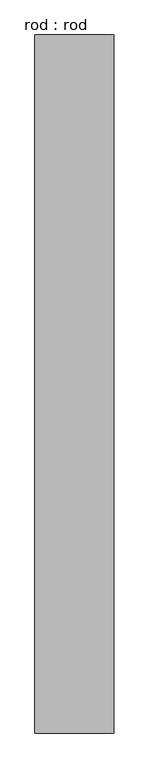
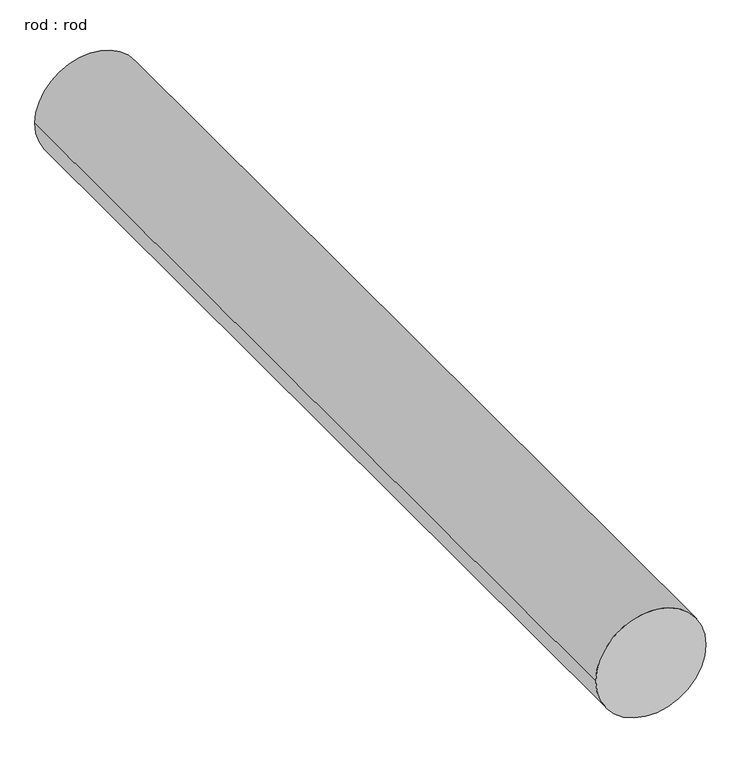
"""IFC4 building model written with IfcOpenShell, lengths in millimetres: proxy geometry, rod : rod."""

from ifc_helpers import new_model, si_unit, point, frame, frame_2d, origin, place, context, project, spatial, circle_curve, trimmed, segment, composite_curve, outline, extrude, source, transform, mapped, element, save


def rod_rod_38694432(model_context):
    return source(origin(), model_context, "Body", "SweptSolid", [
        extrude(outline(composite_curve([segment(trimmed(circle_curve(frame_2d((0.0108462, 0.0)), 200.0), [point((0.0108462, 200.0))], [point((0.0108462, -200.0))], False, "CARTESIAN"), True, "CONTINUOUS"), segment(trimmed(circle_curve(frame_2d((0.0108462, 0.0)), 200.0), [point((0.0108462, -200.0))], [point((0.0108462, 200.0))], False, "CARTESIAN"), True, "CONTINUOUS")], self_intersect=False)), frame((0.0, 2324.8714725, 0.0), z_axis=(0.0, 1.0, 0.0), x_axis=(0.0, 0.0, 1.0)), (0.0, 0.0, 1.0), 3535.7142857),
    ])


if __name__ == "__main__":
    model = new_model("IFC4")
    model_context = context("Model", 3, world=origin())
    ifc_project = project(units=[si_unit("LENGTHUNIT", "METRE", prefix="MILLI")], contexts=[model_context])
    site = spatial("IfcSite", under=ifc_project)
    building = spatial("IfcBuilding", under=site)
    placement = place(None, origin())
    rod_rod_shape = rod_rod_38694432(model_context)
    element("IfcBuildingElementProxy", 1, Name="rod : rod", ObjectType="rod : rod", at=placement, inside=building, context=model_context, shape_type="MappedRepresentation", body=[
        mapped(rod_rod_shape, transform((0.0, 0.0, 0.0), x_axis=(1.0, 0.0, 0.0), y_axis=(0.0, 1.0, 0.0), z_axis=(0.0, 0.0, 1.0))),
    ])
    save(model, "model.ifc")

# Revit data of these elements
# Type "rod : rod"
#   Default Elevation = 0
